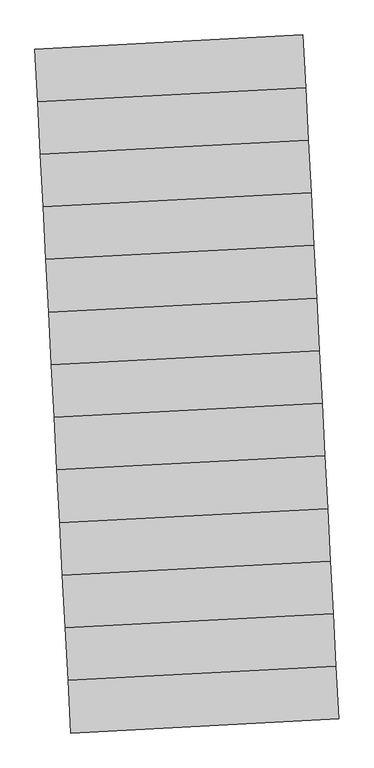
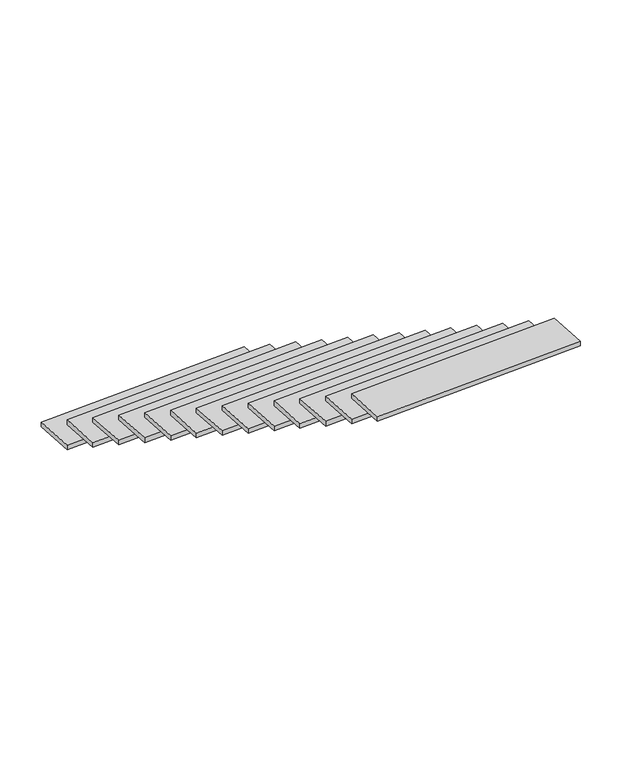
"""IFC4 building model written with IfcOpenShell, lengths in millimetres: stair flight geometry."""

from ifc_helpers import new_model, si_unit, frame, origin, place, context, project, spatial, polyline, outline, extrude, source, transform, mapped, element, save


def stair_flight_a1ef9462(model_context):
    return source(origin(), model_context, "Body", "SweptSolid", [
        extrude(outline(polyline([(25892.6158584, 15125.08554), (24519.5002481, 15053.1236002), (24505.3695399, 15322.7535746), (25878.4851502, 15394.7155144), (25892.6158584, 15125.08554)])), frame((0.0, 0.0, 1768.0), z_axis=(0.0, 0.0, 1.0), x_axis=(1.0, 0.0, 0.0)), (0.0, 0.0, 1.0), 32.0),
        extrude(outline(polyline([(25906.7465666, 14855.4555657), (24533.6309563, 14783.4936258), (24519.5002481, 15053.1236002), (25892.6158584, 15125.08554), (25906.7465666, 14855.4555657)])), frame((0.0, 0.0, 1943.0), z_axis=(0.0, 0.0, 1.0), x_axis=(1.0, 0.0, 0.0)), (0.0, 0.0, 1.0), 32.0),
        extrude(outline(polyline([(25920.8772748, 14585.8255913), (24547.7616645, 14513.8636514), (24533.6309563, 14783.4936258), (25906.7465666, 14855.4555657), (25920.8772748, 14585.8255913)])), frame((0.0, 0.0, 2118.0), z_axis=(0.0, 0.0, 1.0), x_axis=(1.0, 0.0, 0.0)), (0.0, 0.0, 1.0), 32.0),
        extrude(outline(polyline([(25935.007983, 14316.1956169), (24561.8923727, 14244.2336771), (24547.7616645, 14513.8636514), (25920.8772748, 14585.8255913), (25935.007983, 14316.1956169)])), frame((0.0, 0.0, 2293.0), z_axis=(0.0, 0.0, 1.0), x_axis=(1.0, 0.0, 0.0)), (0.0, 0.0, 1.0), 32.0),
        extrude(outline(polyline([(25949.1386911, 14046.5656425), (24576.0230809, 13974.6037027), (24561.8923727, 14244.2336771), (25935.007983, 14316.1956169), (25949.1386911, 14046.5656425)])), frame((0.0, 0.0, 2468.0), z_axis=(0.0, 0.0, 1.0), x_axis=(1.0, 0.0, 0.0)), (0.0, 0.0, 1.0), 32.0),
        extrude(outline(polyline([(25963.2693993, 13776.9356681), (24590.153789, 13704.9737283), (24576.0230809, 13974.6037027), (25949.1386911, 14046.5656425), (25963.2693993, 13776.9356681)])), frame((0.0, 0.0, 2643.0), z_axis=(0.0, 0.0, 1.0), x_axis=(1.0, 0.0, 0.0)), (0.0, 0.0, 1.0), 32.0),
        extrude(outline(polyline([(25977.4001075, 13507.3056937), (24604.2844972, 13435.3437539), (24590.153789, 13704.9737283), (25963.2693993, 13776.9356681), (25977.4001075, 13507.3056937)])), frame((0.0, 0.0, 2818.0), z_axis=(0.0, 0.0, 1.0), x_axis=(1.0, 0.0, 0.0)), (0.0, 0.0, 1.0), 32.0),
        extrude(outline(polyline([(25991.5308157, 13237.6757194), (24618.4152054, 13165.7137795), (24604.2844972, 13435.3437539), (25977.4001075, 13507.3056937), (25991.5308157, 13237.6757194)])), frame((0.0, 0.0, 2993.0), z_axis=(0.0, 0.0, 1.0), x_axis=(1.0, 0.0, 0.0)), (0.0, 0.0, 1.0), 32.0),
        extrude(outline(polyline([(26005.6615239, 12968.045745), (24632.5459136, 12896.0838051), (24618.4152054, 13165.7137795), (25991.5308157, 13237.6757194), (26005.6615239, 12968.045745)])), frame((0.0, 0.0, 3168.0), z_axis=(0.0, 0.0, 1.0), x_axis=(1.0, 0.0, 0.0)), (0.0, 0.0, 1.0), 32.0),
        extrude(outline(polyline([(26019.7922321, 12698.4157706), (24646.6766218, 12626.4538308), (24632.5459136, 12896.0838051), (26005.6615239, 12968.045745), (26019.7922321, 12698.4157706)])), frame((0.0, 0.0, 3343.0), z_axis=(0.0, 0.0, 1.0), x_axis=(1.0, 0.0, 0.0)), (0.0, 0.0, 1.0), 32.0),
        extrude(outline(polyline([(26033.9229403, 12428.7857962), (24660.80733, 12356.8238564), (24646.6766218, 12626.4538308), (26019.7922321, 12698.4157706), (26033.9229403, 12428.7857962)])), frame((0.0, 0.0, 3518.0), z_axis=(0.0, 0.0, 1.0), x_axis=(1.0, 0.0, 0.0)), (0.0, 0.0, 1.0), 32.0),
        extrude(outline(polyline([(26048.0536484, 12159.1558218), (24674.9380382, 12087.193882), (24660.80733, 12356.8238564), (26033.9229403, 12428.7857962), (26048.0536484, 12159.1558218)])), frame((0.0, 0.0, 3693.0), z_axis=(0.0, 0.0, 1.0), x_axis=(1.0, 0.0, 0.0)), (0.0, 0.0, 1.0), 32.0),
        extrude(outline(polyline([(26062.1843566, 11889.5258474), (24689.0687463, 11817.5639076), (24674.9380382, 12087.193882), (26048.0536484, 12159.1558218), (26062.1843566, 11889.5258474)])), frame((0.0, 0.0, 3868.0), z_axis=(0.0, 0.0, 1.0), x_axis=(1.0, 0.0, 0.0)), (0.0, 0.0, 1.0), 32.0),
    ])


if __name__ == "__main__":
    model = new_model("IFC4")
    model_context = context("Model", 3, world=origin())
    ifc_project = project(units=[si_unit("LENGTHUNIT", "METRE", prefix="MILLI")], contexts=[model_context])
    site = spatial("IfcSite", under=ifc_project)
    building = spatial("IfcBuilding", under=site)
    placement = place(None, origin())
    stair_flight_shape = stair_flight_a1ef9462(model_context)
    element("IfcStairFlight", 1, at=placement, inside=building, context=model_context, shape_type="MappedRepresentation", body=[
        mapped(stair_flight_shape, transform((0.0, 0.0, 0.0), x_axis=(1.0, 0.0, 0.0), y_axis=(0.0, 1.0, 0.0), z_axis=(0.0, 0.0, 1.0))),
    ])
    save(model, "model.ifc")

# Revit data of these elements
# Element 1 (IfcStairFlight)
#   Materials on its faces: "철강"
# Materials
#   "철강": class "Generic", colour RGB 143 142 141, transparency 0, Description = "철골+가공조립+세우기", Cost = 0
